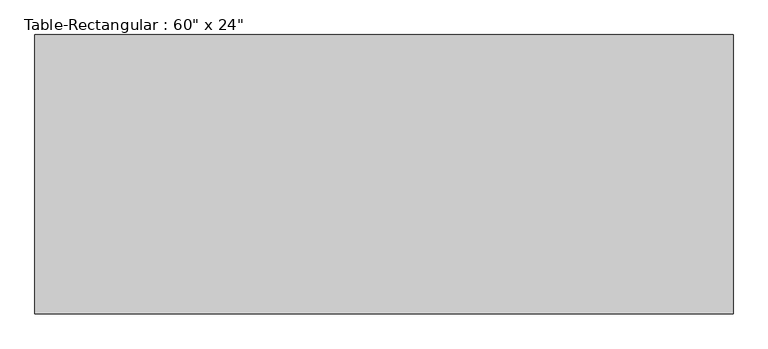
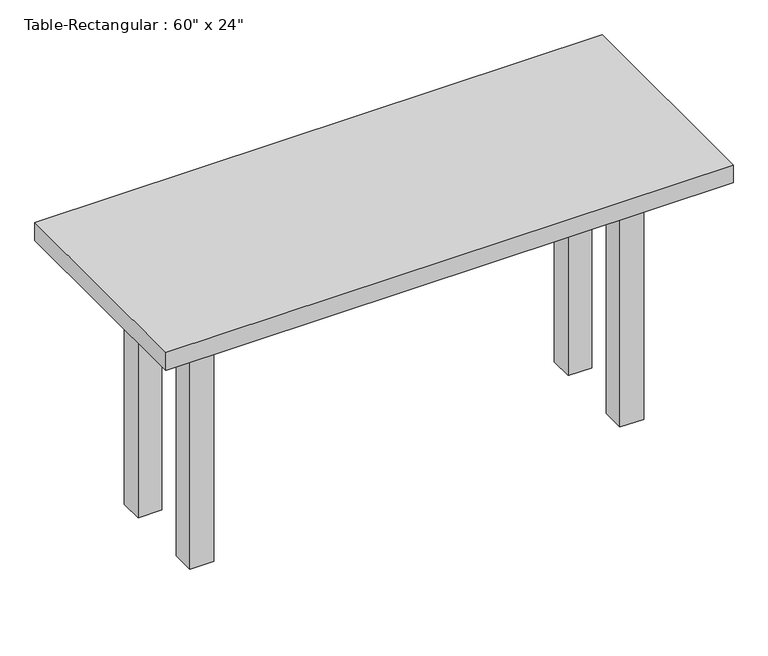
"""IFC4 building model written with IfcOpenShell, lengths in millimetres: furniture geometry."""

from ifc_helpers import new_model, si_unit, frame, origin, origin_with_axes, place, context, project, spatial, polyline, outline, extrude, source, transform, mapped, element, save


def furniture_3e3a90ab(model_context):
    return source(origin(), model_context, "Body", "SweptSolid", [
        extrude(outline(polyline([(546.1, 114.3), (546.1, 88.9), (-546.1, 88.9), (-546.1, 114.3), (546.1, 114.3)])), frame((0.0, 0.0, 609.6), z_axis=(0.0, 0.0, 1.0), x_axis=(1.0, 0.0, 0.0)), (0.0, 0.0, 1.0), 101.6),
        extrude(outline(polyline([(546.1, -114.3), (-546.1, -114.3), (-546.1, -88.9), (546.1, -88.9), (546.1, -114.3)])), frame((0.0, 0.0, 609.6), z_axis=(0.0, 0.0, 1.0), x_axis=(1.0, 0.0, 0.0)), (0.0, 0.0, 1.0), 101.6),
        extrude(outline(polyline([(-558.8, -88.9), (-584.2, -88.9), (-584.2, 88.9), (-558.8, 88.9), (-558.8, -88.9)])), frame((0.0, 0.0, 609.6), z_axis=(0.0, 0.0, 1.0), x_axis=(1.0, 0.0, 0.0)), (0.0, 0.0, 1.0), 101.6),
        extrude(outline(polyline([(558.8, -88.9), (558.8, 88.9), (584.2, 88.9), (584.2, -88.9), (558.8, -88.9)])), frame((0.0, 0.0, 609.6), z_axis=(0.0, 0.0, 1.0), x_axis=(1.0, 0.0, 0.0)), (0.0, 0.0, 1.0), 101.6),
        extrude(outline(polyline([(762.0, 304.8), (762.0, -304.8), (-762.0, -304.8), (-762.0, 304.8), (762.0, 304.8)])), frame((0.0, 0.0, 711.2), z_axis=(0.0, 0.0, 1.0), x_axis=(1.0, 0.0, 0.0)), (0.0, 0.0, 1.0), 50.8),
        extrude(outline(polyline([(-546.1, 152.4), (-546.1, 88.9), (-609.6, 88.9), (-609.6, 152.4), (-546.1, 152.4)])), origin_with_axes(), (0.0, 0.0, 1.0), 711.2),
        extrude(outline(polyline([(546.1, 152.4), (609.6, 152.4), (609.6, 88.9), (546.1, 88.9), (546.1, 152.4)])), origin_with_axes(), (0.0, 0.0, 1.0), 711.2),
        extrude(outline(polyline([(-546.1, -152.4), (-609.6, -152.4), (-609.6, -88.9), (-546.1, -88.9), (-546.1, -152.4)])), origin_with_axes(), (0.0, 0.0, 1.0), 711.2),
        extrude(outline(polyline([(546.1, -152.4), (546.1, -88.9), (609.6, -88.9), (609.6, -152.4), (546.1, -152.4)])), origin_with_axes(), (0.0, 0.0, 1.0), 711.2),
    ])


if __name__ == "__main__":
    model = new_model("IFC4")
    model_context = context("Model", 3, world=origin())
    ifc_project = project(units=[si_unit("LENGTHUNIT", "METRE", prefix="MILLI")], contexts=[model_context])
    site = spatial("IfcSite", under=ifc_project)
    building = spatial("IfcBuilding", under=site)
    placement = place(None, origin())
    furniture_shape = furniture_3e3a90ab(model_context)
    element("IfcFurniture", 1, ObjectType="Table-Rectangular : 60\" x 24\"", at=placement, inside=building, context=model_context, shape_type="MappedRepresentation", body=[
        mapped(furniture_shape, transform((0.0, 0.0, 0.0), x_axis=(1.0, 0.0, 0.0), y_axis=(0.0, 1.0, 0.0), z_axis=(0.0, 0.0, 1.0))),
    ])
    save(model, "model.ifc")

# Revit data of these elements
# Type "Table-Rectangular : 60\" x 24\""
#   Model = "Desk"
#   Manufacturer = "Acme Funriture"
#   Assembly Code = "E2020200"
#   Height = 2' - 6"
#   Length = 5' - 0"
#   Width = 2' - 0"
#   Base Material = Birch
#   Top Material = Laminate, Blue, Matte
#   Default Elevation = 0
# Element 1 (IfcFurniture, "Table-Rectangular : 60\" x 24\"")
#   Materials on its faces: "Birch", "Laminate, Blue, Matte"
# Materials
#   "Birch": class "Wood", colour RGB 172 132 95, transparency 0, Description = "Betula Alleghaniensis", Cost = 0
#   "Laminate, Blue, Matte": class "Plastic", colour RGB 85 101 155, transparency 0, Description = "Plastic Laminate - Blue, Matte", Cost = 0
